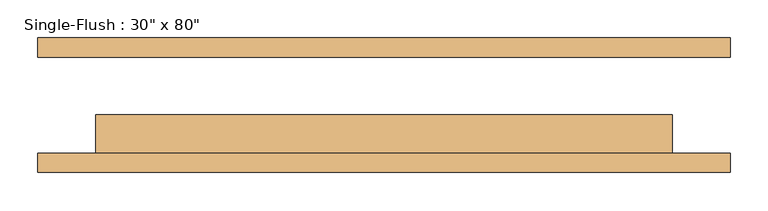
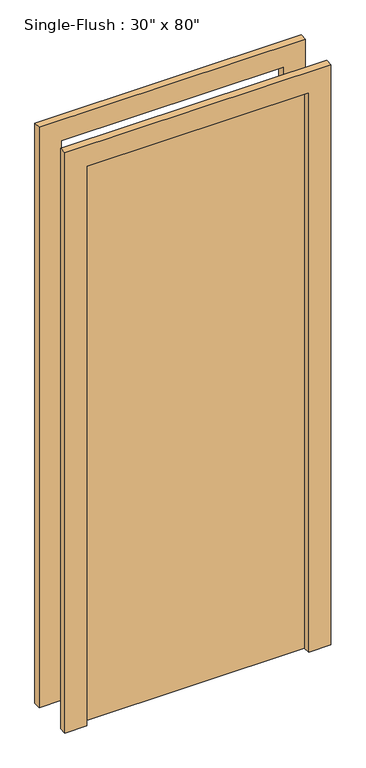
"""IFC4 building model written with IfcOpenShell, lengths in millimetres: door geometry."""

import ifcopenshell
import ifcopenshell.guid

model = None  # the IFC model being written
_history = None  # IfcOwnerHistory: only IFC2X3 demands one
_inside = {}  # id of a spatial element -> (the spatial element, [elements in it])
_under = {}  # id of a project, library or spatial element -> (it, [spatial elements below it])
_declared = {}  # id of a project -> (the project, [libraries it declares])
_typed = {}  # id of a type object -> (the type object, [elements of that type])
_made_of = {}  # id of a material, layer set ... -> (it, [elements and type objects made of it])


def new_model(schema):
    """Start an empty IFC model of exactly this schema.

    Asked for "IFC4X3", IfcOpenShell would pick the latest addendum, in which some entities
    have other attributes; the version numbers below select the first issue.
    IFC2X3 requires an IfcOwnerHistory on every rooted entity: one is made here for all.
    """
    global model, _history
    if schema == "IFC4X3":
        model = ifcopenshell.file(schema_version=(4, 3, 0, 0))
    else:
        model = ifcopenshell.file(schema=schema)
    _inside.clear()
    _under.clear()
    _declared.clear()
    _typed.clear()
    _made_of.clear()
    _history = None
    if model.schema == "IFC2X3":
        org = make("IfcOrganization", Name="unknown")
        user = make(
            "IfcPersonAndOrganization",
            ThePerson=make("IfcPerson", FamilyName="unknown"),
            TheOrganization=org,
        )
        app = make(
            "IfcApplication",
            ApplicationDeveloper=org,
            Version="unknown",
            ApplicationFullName="unknown",
            ApplicationIdentifier="unknown",
        )
        _history = make(
            "IfcOwnerHistory",
            OwningUser=user,
            OwningApplication=app,
            ChangeAction="ADDED",
            CreationDate=0,
        )
    return model


def make(cls, **values):
    """One entity of the class cls with the attributes given. An attribute that is None is left unset."""
    return model.create_entity(
        cls, **{name: value for name, value in values.items() if value is not None}
    )


def rooted(cls, **values):
    """An entity with a GlobalId (a new one), such as an element, a storey or a relation."""
    return make(cls, GlobalId=ifcopenshell.guid.new(), OwnerHistory=_history, **values)


def si_unit(unit_type, name, prefix=None):
    """IfcSIUnit, for example si_unit("LENGTHUNIT", "METRE", prefix="MILLI")."""
    return make("IfcSIUnit", UnitType=unit_type, Prefix=prefix, Name=name)


def assignment(units):
    """IfcUnitAssignment: the units of a project."""
    return None if units is None else make("IfcUnitAssignment", Units=units)


def point(xyz):
    """IfcCartesianPoint."""
    return None if xyz is None else make("IfcCartesianPoint", Coordinates=xyz)


def direction(xyz):
    """IfcDirection."""
    return None if xyz is None else make("IfcDirection", DirectionRatios=xyz)


def frame(location, z_axis=None, x_axis=None):
    """IfcAxis2Placement3D, a coordinate frame: its origin and axes. An axis left out is left unset."""
    return make(
        "IfcAxis2Placement3D",
        Location=point(location),
        Axis=direction(z_axis),
        RefDirection=direction(x_axis),
    )


def origin():
    """The frame at (0, 0, 0) with its axes left unset."""
    return frame((0.0, 0.0, 0.0))


def origin_with_axes():
    """The frame at (0, 0, 0) with the z axis (0, 0, 1) and the x axis (1, 0, 0) written out."""
    return frame((0.0, 0.0, 0.0), z_axis=(0.0, 0.0, 1.0), x_axis=(1.0, 0.0, 0.0))


def place(relative_to, where):
    """IfcLocalPlacement: puts the frame where relative to a parent placement (None: the world)."""
    return make(
        "IfcLocalPlacement", PlacementRelTo=relative_to, RelativePlacement=where
    )


def context(
    kind, dimensions, precision=None, world=None, true_north=None, identifier=None
):
    """IfcGeometricRepresentationContext, for example the 3D "Model" context."""
    return make(
        "IfcGeometricRepresentationContext",
        ContextIdentifier=identifier,
        ContextType=kind,
        CoordinateSpaceDimension=dimensions,
        Precision=precision,
        WorldCoordinateSystem=world,
        TrueNorth=true_north,
    )


def project(units=None, contexts=None):
    """IfcProject with its units and contexts."""
    return rooted(
        "IfcProject",
        Name="project",
        RepresentationContexts=contexts,
        UnitsInContext=assignment(units),
    )


def spatial(cls, under=None, at=None, **own):
    """A site, building, storey or space (cls), placed at a placement, below another one or the project."""
    s = rooted(cls, ObjectPlacement=at, **own)
    if under is not None:
        _under.setdefault(under.id(), (under, []))[1].append(s)
    return s


def polyline(points):
    """IfcPolyline through the points."""
    return make("IfcPolyline", Points=[point(p) for p in points])


def outline(outer, holes=None, kind="AREA"):
    """IfcArbitraryClosedProfileDef: a profile drawn as a closed curve; with holes, ...WithVoids."""
    if holes is None:
        return make("IfcArbitraryClosedProfileDef", ProfileType=kind, OuterCurve=outer)
    return make(
        "IfcArbitraryProfileDefWithVoids",
        ProfileType=kind,
        OuterCurve=outer,
        InnerCurves=holes,
    )


def extrude(swept, where, along, depth):
    """IfcExtrudedAreaSolid: the profile swept, set in the frame where, extruded along a direction by depth."""
    return make(
        "IfcExtrudedAreaSolid",
        SweptArea=swept,
        Position=where,
        ExtrudedDirection=direction(along),
        Depth=depth,
    )


def shape(context_of_items, identifier, shape_type, items):
    """IfcShapeRepresentation: the items that make up one representation, for example the "Body"."""
    return make(
        "IfcShapeRepresentation",
        ContextOfItems=context_of_items,
        RepresentationIdentifier=identifier,
        RepresentationType=shape_type,
        Items=items,
    )


def source(mapping_origin, context_of_items, identifier, shape_type, items):
    """IfcRepresentationMap: a shape defined once, which mapped items show again and again."""
    return make(
        "IfcRepresentationMap",
        MappingOrigin=mapping_origin,
        MappedRepresentation=shape(context_of_items, identifier, shape_type, items),
    )


def transform(
    local_origin,
    x_axis=None,
    y_axis=None,
    z_axis=None,
    scale=None,
    scale2=None,
    scale3=None,
    uniform=True,
):
    """IfcCartesianTransformationOperator3D, or its non-uniform kind. x_axis, y_axis, z_axis: its Axis1, 2, 3."""
    if uniform:
        return make(
            "IfcCartesianTransformationOperator3D",
            Axis1=direction(x_axis),
            Axis2=direction(y_axis),
            LocalOrigin=point(local_origin),
            Scale=scale,
            Axis3=direction(z_axis),
        )
    return make(
        "IfcCartesianTransformationOperator3DnonUniform",
        Axis1=direction(x_axis),
        Axis2=direction(y_axis),
        LocalOrigin=point(local_origin),
        Scale=scale,
        Axis3=direction(z_axis),
        Scale2=scale2,
        Scale3=scale3,
    )


def mapped(mapping_source, mapping_target):
    """IfcMappedItem: shows the shape of a source again, moved by a transform."""
    return make(
        "IfcMappedItem", MappingSource=mapping_source, MappingTarget=mapping_target
    )


def made_of(thing, what):
    """Note that an element or type object is made of a material, layer set ...; save() writes the relation."""
    if what is not None:
        _made_of.setdefault(what.id(), (what, []))[1].append(thing)
    return thing


def element(
    cls,
    number,
    at=None,
    inside=None,
    cuts=None,
    type_object=None,
    material=None,
    context=None,
    identifier="Body",
    shape_type=None,
    held_by="IfcProductDefinitionShape",
    body=None,
    shapes=None,
    **own,
):
    """One element of the class cls, such as IfcWall. Its Tag is "e" and its number.

    at: its placement. inside: the storey or other place that contains it. cuts: it is an
    opening in that element (IfcRelVoidsElement). A single representation is given by context,
    identifier, shape_type and body (its items); several are given by shapes. held_by: the class
    of the entity that holds the representations. save() writes the other relations.
    """
    e = rooted(cls, Tag="e%d" % number, ObjectPlacement=at, **own)
    if body is not None:
        shapes = [shape(context, identifier, shape_type, body)]
    if shapes is not None:
        e.Representation = make(held_by, Representations=shapes)
    if inside is not None:
        _inside.setdefault(inside.id(), (inside, []))[1].append(e)
    if cuts is not None:
        rooted(
            "IfcRelVoidsElement", RelatingBuildingElement=cuts, RelatedOpeningElement=e
        )
    if type_object is not None:
        _typed.setdefault(type_object.id(), (type_object, []))[1].append(e)
    return made_of(e, material)


def aggregate(whole, parts):
    """IfcRelAggregates: a whole, such as a stair, and the parts it consists of."""
    return rooted("IfcRelAggregates", RelatingObject=whole, RelatedObjects=parts)


def save(model, path):
    """Write the relations noted so far, then the file.

    IfcRelAggregates (storeys below a building ...), IfcRelContainedInSpatialStructure (elements
    in a storey), IfcRelDefinesByType, IfcRelAssociatesMaterial and IfcRelDeclares: one each for
    every whole, place, type object, material and project.
    """
    for whole, parts in _under.values():
        aggregate(whole, parts)
    for where, things in _inside.values():
        rooted(
            "IfcRelContainedInSpatialStructure",
            RelatedElements=things,
            RelatingStructure=where,
        )
    for kind, things in _typed.values():
        rooted("IfcRelDefinesByType", RelatedObjects=things, RelatingType=kind)
    for what, things in _made_of.values():
        rooted("IfcRelAssociatesMaterial", RelatedObjects=things, RelatingMaterial=what)
    for by, libraries in _declared.values():
        rooted("IfcRelDeclares", RelatingContext=by, RelatedDefinitions=libraries)
    model.write(path)


def door_e00f436c(model_context):
    return source(origin(), model_context, "Body", "SweptSolid", [
        extrude(outline(polyline([(2108.2, -457.2), (0.0, -457.2), (0.0, -381.0), (2032.0, -381.0), (2032.0, 381.0), (0.0, 381.0), (0.0, 457.2), (2108.2, 457.2), (2108.2, -457.2)])), frame((0.0, -88.9, 0.0), z_axis=(0.0, 1.0, 0.0), x_axis=(0.0, 0.0, 1.0)), (0.0, 0.0, 1.0), 25.4),
        extrude(outline(polyline([(2108.2, 457.2), (2108.2, -457.2), (0.0, -457.2), (0.0, -381.0), (2032.0, -381.0), (2032.0, 381.0), (0.0, 381.0), (0.0, 457.2), (2108.2, 457.2)])), frame((0.0, 63.5, 0.0), z_axis=(0.0, 1.0, 0.0), x_axis=(0.0, 0.0, 1.0)), (0.0, 0.0, 1.0), 25.4),
        extrude(outline(polyline([(381.0, -12.7), (381.0, -63.5), (-381.0, -63.5), (-381.0, -12.7), (381.0, -12.7)])), origin_with_axes(), (0.0, 0.0, 1.0), 2032.0),
    ])


if __name__ == "__main__":
    model = new_model("IFC4")
    model_context = context("Model", 3, world=origin())
    ifc_project = project(units=[si_unit("LENGTHUNIT", "METRE", prefix="MILLI")], contexts=[model_context])
    site = spatial("IfcSite", under=ifc_project)
    building = spatial("IfcBuilding", under=site)
    placement = place(None, origin())
    door_shape = door_e00f436c(model_context)
    element("IfcDoor", 1, ObjectType="Single-Flush : 30\" x 80\"", at=placement, inside=building, context=model_context, shape_type="MappedRepresentation", body=[
        mapped(door_shape, transform((0.0, 0.0, 0.0), x_axis=(1.0, 0.0, 0.0), y_axis=(0.0, 1.0, 0.0), z_axis=(0.0, 0.0, 1.0))),
    ])
    save(model, "model.ifc")

# Revit data of these elements
# Type "Single-Flush : 30\" x 80\""
#   Type Mark = "5"
#   Construction Type Id = "MDOOR"
#   Assembly Code = "C1020"
#   Analytic Construction = "Metal"
#   Thickness = 0' - 2"
#   Heat Transfer Coefficient (U) = 0.651978 BTU/(h·ft²·°F)
#   Height = 6' - 8"
#   Trim Projection Ext = 0' - 1"
#   Trim Projection Int = 0' - 1"
#   Trim Width = 0' - 3"
#   Width = 2' - 6"
#   Define Thermal Properties by = 1
#   Define Thermal Properties by = 1
#   Door Material = Door - Panel
#   Frame Material = Door - Frame
#   Visual Light Transmittance = 0
#   Solar Heat Gain Coefficient = 0
#   Function = (empty or 0)
#   Wall Closure = (empty or 0)
# Element 1 (IfcDoor, "Single-Flush : 30\" x 80\"")
#   Materials on its faces: "Door - Frame", "Door - Panel"
# Materials
#   "Door - Panel": class "Wood", colour RGB 210 159 95, transparency 0, Cost = 0
#   "Door - Frame": class "Miscellaneous", colour RGB 118 70 51, transparency 0, Cost = 0
